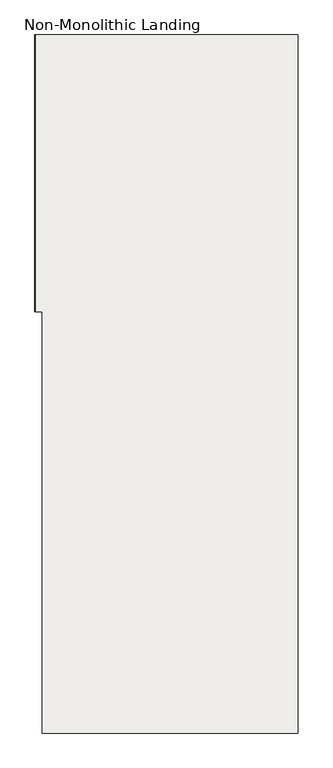
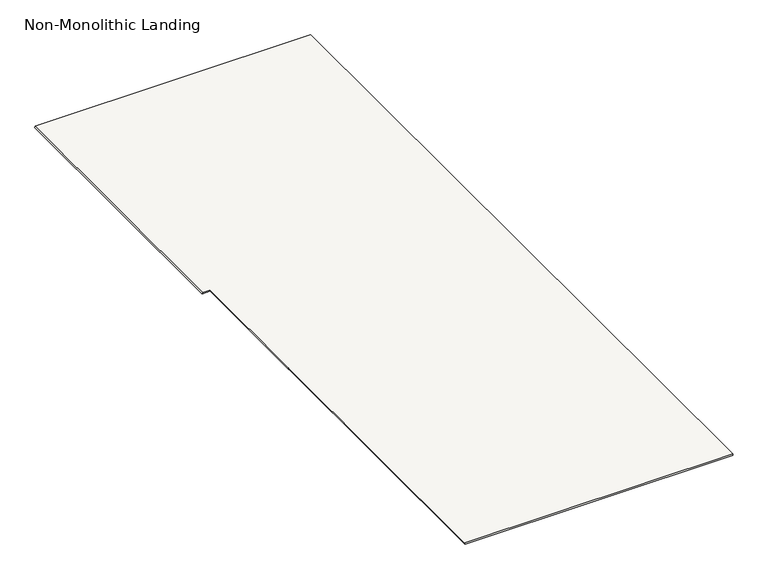
"""IFC4 building model written with IfcOpenShell, lengths in millimetres: slab geometry, Non-Monolithic Landing."""

from ifc_helpers import new_model, si_unit, origin, place, context, project, spatial, faceted_brep, source, transform, mapped, element, save


def non_monolithic_landing_d1c94219(model_context):
    return source(origin(), model_context, "Body", "Brep", [
        faceted_brep([(16318.9409643, 13220.4345331, 6222.2222222), (16318.0972143, 13220.4345331, 6216.2222222), (16318.0972143, 12030.4345331, 6216.2222222), (16318.9409643, 12030.4345331, 6222.2222222), (16350.0, 10220.4345331, 6222.2222222), (17450.0, 10220.4345331, 6222.2222222), (17450.0, 13220.4345331, 6222.2222222), (16350.0, 13220.4345331, 6222.2222222), (16350.0, 12030.4345331, 6222.2222222), (16350.0, 11470.4345331, 6222.2222222), (17450.0, 13220.4345331, 6216.2222222), (17450.0, 10220.4345331, 6216.2222222), (16350.84375, 10220.4345331, 6216.2222222), (16350.84375, 11470.4345331, 6216.2222222), (16350.0, 11470.4345331, 6216.2222222), (16350.0, 12030.4345331, 6216.2222222), (16350.0, 13220.4345331, 6216.2222222)], [[[0, 1, 2, 3]], [[4, 5, 6, 7, 0, 3, 8, 9]], [[10, 11, 12, 13, 14, 15, 2, 1, 16]], [[9, 8, 15, 14]], [[0, 7, 16, 1]], [[7, 6, 10, 16]], [[6, 5, 11, 10]], [[5, 4, 12, 11]], [[13, 9, 14]], [[9, 13, 12, 4]], [[8, 3, 2, 15]]]),
    ])


if __name__ == "__main__":
    model = new_model("IFC4")
    model_context = context("Model", 3, world=origin())
    ifc_project = project(units=[si_unit("LENGTHUNIT", "METRE", prefix="MILLI")], contexts=[model_context])
    site = spatial("IfcSite", under=ifc_project)
    building = spatial("IfcBuilding", under=site)
    placement = place(None, origin())
    non_monolithic_landing_shape = non_monolithic_landing_d1c94219(model_context)
    element("IfcSlab", 1, ObjectType="Non-Monolithic Landing", at=placement, inside=building, context=model_context, shape_type="MappedRepresentation", body=[
        mapped(non_monolithic_landing_shape, transform((0.0, 0.0, 0.0), x_axis=(1.0, 0.0, 0.0), y_axis=(0.0, 1.0, 0.0), z_axis=(0.0, 0.0, 1.0))),
    ])
    save(model, "model.ifc")

# Revit data of these elements
# Element 1 (IfcSlab, "Non-Monolithic Landing")
#   Materials on its faces: "Steel, Paint Finish, Dark Gray"
# Materials
#   "Steel, Paint Finish, Dark Gray": class "Metal", colour RGB 89 89 89, transparency 0, Description = "Steel, paint finish, dark gray, glossy", Cost = 0
